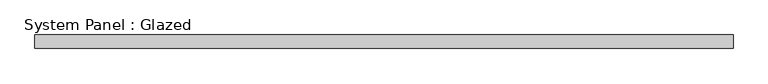
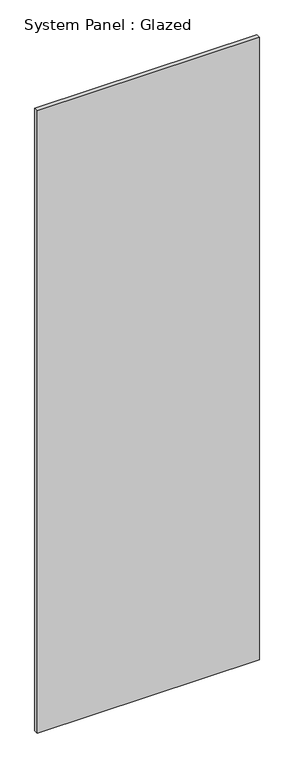
"""IFC4 building model written with IfcOpenShell, lengths in millimetres: plate geometry, System Panel : Glazed."""

import ifcopenshell
import ifcopenshell.guid

model = None  # the IFC model being written
_history = None  # IfcOwnerHistory: only IFC2X3 demands one
_inside = {}  # id of a spatial element -> (the spatial element, [elements in it])
_under = {}  # id of a project, library or spatial element -> (it, [spatial elements below it])
_declared = {}  # id of a project -> (the project, [libraries it declares])
_typed = {}  # id of a type object -> (the type object, [elements of that type])
_made_of = {}  # id of a material, layer set ... -> (it, [elements and type objects made of it])


def new_model(schema):
    """Start an empty IFC model of exactly this schema.

    Asked for "IFC4X3", IfcOpenShell would pick the latest addendum, in which some entities
    have other attributes; the version numbers below select the first issue.
    IFC2X3 requires an IfcOwnerHistory on every rooted entity: one is made here for all.
    """
    global model, _history
    if schema == "IFC4X3":
        model = ifcopenshell.file(schema_version=(4, 3, 0, 0))
    else:
        model = ifcopenshell.file(schema=schema)
    _inside.clear()
    _under.clear()
    _declared.clear()
    _typed.clear()
    _made_of.clear()
    _history = None
    if model.schema == "IFC2X3":
        org = make("IfcOrganization", Name="unknown")
        user = make(
            "IfcPersonAndOrganization",
            ThePerson=make("IfcPerson", FamilyName="unknown"),
            TheOrganization=org,
        )
        app = make(
            "IfcApplication",
            ApplicationDeveloper=org,
            Version="unknown",
            ApplicationFullName="unknown",
            ApplicationIdentifier="unknown",
        )
        _history = make(
            "IfcOwnerHistory",
            OwningUser=user,
            OwningApplication=app,
            ChangeAction="ADDED",
            CreationDate=0,
        )
    return model


def make(cls, **values):
    """One entity of the class cls with the attributes given. An attribute that is None is left unset."""
    return model.create_entity(
        cls, **{name: value for name, value in values.items() if value is not None}
    )


def rooted(cls, **values):
    """An entity with a GlobalId (a new one), such as an element, a storey or a relation."""
    return make(cls, GlobalId=ifcopenshell.guid.new(), OwnerHistory=_history, **values)


def si_unit(unit_type, name, prefix=None):
    """IfcSIUnit, for example si_unit("LENGTHUNIT", "METRE", prefix="MILLI")."""
    return make("IfcSIUnit", UnitType=unit_type, Prefix=prefix, Name=name)


def assignment(units):
    """IfcUnitAssignment: the units of a project."""
    return None if units is None else make("IfcUnitAssignment", Units=units)


def point(xyz):
    """IfcCartesianPoint."""
    return None if xyz is None else make("IfcCartesianPoint", Coordinates=xyz)


def direction(xyz):
    """IfcDirection."""
    return None if xyz is None else make("IfcDirection", DirectionRatios=xyz)


def frame(location, z_axis=None, x_axis=None):
    """IfcAxis2Placement3D, a coordinate frame: its origin and axes. An axis left out is left unset."""
    return make(
        "IfcAxis2Placement3D",
        Location=point(location),
        Axis=direction(z_axis),
        RefDirection=direction(x_axis),
    )


def origin():
    """The frame at (0, 0, 0) with its axes left unset."""
    return frame((0.0, 0.0, 0.0))


def origin_with_axes():
    """The frame at (0, 0, 0) with the z axis (0, 0, 1) and the x axis (1, 0, 0) written out."""
    return frame((0.0, 0.0, 0.0), z_axis=(0.0, 0.0, 1.0), x_axis=(1.0, 0.0, 0.0))


def place(relative_to, where):
    """IfcLocalPlacement: puts the frame where relative to a parent placement (None: the world)."""
    return make(
        "IfcLocalPlacement", PlacementRelTo=relative_to, RelativePlacement=where
    )


def context(
    kind, dimensions, precision=None, world=None, true_north=None, identifier=None
):
    """IfcGeometricRepresentationContext, for example the 3D "Model" context."""
    return make(
        "IfcGeometricRepresentationContext",
        ContextIdentifier=identifier,
        ContextType=kind,
        CoordinateSpaceDimension=dimensions,
        Precision=precision,
        WorldCoordinateSystem=world,
        TrueNorth=true_north,
    )


def project(units=None, contexts=None):
    """IfcProject with its units and contexts."""
    return rooted(
        "IfcProject",
        Name="project",
        RepresentationContexts=contexts,
        UnitsInContext=assignment(units),
    )


def spatial(cls, under=None, at=None, **own):
    """A site, building, storey or space (cls), placed at a placement, below another one or the project."""
    s = rooted(cls, ObjectPlacement=at, **own)
    if under is not None:
        _under.setdefault(under.id(), (under, []))[1].append(s)
    return s


def polyline(points):
    """IfcPolyline through the points."""
    return make("IfcPolyline", Points=[point(p) for p in points])


def outline(outer, holes=None, kind="AREA"):
    """IfcArbitraryClosedProfileDef: a profile drawn as a closed curve; with holes, ...WithVoids."""
    if holes is None:
        return make("IfcArbitraryClosedProfileDef", ProfileType=kind, OuterCurve=outer)
    return make(
        "IfcArbitraryProfileDefWithVoids",
        ProfileType=kind,
        OuterCurve=outer,
        InnerCurves=holes,
    )


def extrude(swept, where, along, depth):
    """IfcExtrudedAreaSolid: the profile swept, set in the frame where, extruded along a direction by depth."""
    return make(
        "IfcExtrudedAreaSolid",
        SweptArea=swept,
        Position=where,
        ExtrudedDirection=direction(along),
        Depth=depth,
    )


def shape(context_of_items, identifier, shape_type, items):
    """IfcShapeRepresentation: the items that make up one representation, for example the "Body"."""
    return make(
        "IfcShapeRepresentation",
        ContextOfItems=context_of_items,
        RepresentationIdentifier=identifier,
        RepresentationType=shape_type,
        Items=items,
    )


def source(mapping_origin, context_of_items, identifier, shape_type, items):
    """IfcRepresentationMap: a shape defined once, which mapped items show again and again."""
    return make(
        "IfcRepresentationMap",
        MappingOrigin=mapping_origin,
        MappedRepresentation=shape(context_of_items, identifier, shape_type, items),
    )


def transform(
    local_origin,
    x_axis=None,
    y_axis=None,
    z_axis=None,
    scale=None,
    scale2=None,
    scale3=None,
    uniform=True,
):
    """IfcCartesianTransformationOperator3D, or its non-uniform kind. x_axis, y_axis, z_axis: its Axis1, 2, 3."""
    if uniform:
        return make(
            "IfcCartesianTransformationOperator3D",
            Axis1=direction(x_axis),
            Axis2=direction(y_axis),
            LocalOrigin=point(local_origin),
            Scale=scale,
            Axis3=direction(z_axis),
        )
    return make(
        "IfcCartesianTransformationOperator3DnonUniform",
        Axis1=direction(x_axis),
        Axis2=direction(y_axis),
        LocalOrigin=point(local_origin),
        Scale=scale,
        Axis3=direction(z_axis),
        Scale2=scale2,
        Scale3=scale3,
    )


def mapped(mapping_source, mapping_target):
    """IfcMappedItem: shows the shape of a source again, moved by a transform."""
    return make(
        "IfcMappedItem", MappingSource=mapping_source, MappingTarget=mapping_target
    )


def made_of(thing, what):
    """Note that an element or type object is made of a material, layer set ...; save() writes the relation."""
    if what is not None:
        _made_of.setdefault(what.id(), (what, []))[1].append(thing)
    return thing


def element(
    cls,
    number,
    at=None,
    inside=None,
    cuts=None,
    type_object=None,
    material=None,
    context=None,
    identifier="Body",
    shape_type=None,
    held_by="IfcProductDefinitionShape",
    body=None,
    shapes=None,
    **own,
):
    """One element of the class cls, such as IfcWall. Its Tag is "e" and its number.

    at: its placement. inside: the storey or other place that contains it. cuts: it is an
    opening in that element (IfcRelVoidsElement). A single representation is given by context,
    identifier, shape_type and body (its items); several are given by shapes. held_by: the class
    of the entity that holds the representations. save() writes the other relations.
    """
    e = rooted(cls, Tag="e%d" % number, ObjectPlacement=at, **own)
    if body is not None:
        shapes = [shape(context, identifier, shape_type, body)]
    if shapes is not None:
        e.Representation = make(held_by, Representations=shapes)
    if inside is not None:
        _inside.setdefault(inside.id(), (inside, []))[1].append(e)
    if cuts is not None:
        rooted(
            "IfcRelVoidsElement", RelatingBuildingElement=cuts, RelatedOpeningElement=e
        )
    if type_object is not None:
        _typed.setdefault(type_object.id(), (type_object, []))[1].append(e)
    return made_of(e, material)


def aggregate(whole, parts):
    """IfcRelAggregates: a whole, such as a stair, and the parts it consists of."""
    return rooted("IfcRelAggregates", RelatingObject=whole, RelatedObjects=parts)


def save(model, path):
    """Write the relations noted so far, then the file.

    IfcRelAggregates (storeys below a building ...), IfcRelContainedInSpatialStructure (elements
    in a storey), IfcRelDefinesByType, IfcRelAssociatesMaterial and IfcRelDeclares: one each for
    every whole, place, type object, material and project.
    """
    for whole, parts in _under.values():
        aggregate(whole, parts)
    for where, things in _inside.values():
        rooted(
            "IfcRelContainedInSpatialStructure",
            RelatedElements=things,
            RelatingStructure=where,
        )
    for kind, things in _typed.values():
        rooted("IfcRelDefinesByType", RelatedObjects=things, RelatingType=kind)
    for what, things in _made_of.values():
        rooted("IfcRelAssociatesMaterial", RelatedObjects=things, RelatingMaterial=what)
    for by, libraries in _declared.values():
        rooted("IfcRelDeclares", RelatingContext=by, RelatedDefinitions=libraries)
    model.write(path)


def system_panel_glazed_f91df05e(model_context):
    return source(origin(), model_context, "Body", "SweptSolid", [
        extrude(outline(polyline([(660.033654, 19.05), (-660.033654, 19.05), (-660.033654, 44.45), (660.033654, 44.45), (660.033654, 19.05)])), origin_with_axes(), (0.0, 0.0, 1.0), 3908.2835741),
    ])


if __name__ == "__main__":
    model = new_model("IFC4")
    model_context = context("Model", 3, world=origin())
    ifc_project = project(units=[si_unit("LENGTHUNIT", "METRE", prefix="MILLI")], contexts=[model_context])
    site = spatial("IfcSite", under=ifc_project)
    building = spatial("IfcBuilding", under=site)
    placement = place(None, origin())
    system_panel_glazed_shape = system_panel_glazed_f91df05e(model_context)
    element("IfcPlate", 1, ObjectType="System Panel : Glazed", at=placement, inside=building, context=model_context, shape_type="MappedRepresentation", body=[
        mapped(system_panel_glazed_shape, transform((0.0, 0.0, 0.0), x_axis=(1.0, 0.0, 0.0), y_axis=(0.0, 1.0, 0.0), z_axis=(0.0, 0.0, 1.0))),
    ])
    save(model, "model.ifc")

# Revit data of these elements
# Type "System Panel : Glazed"
#   Construction Type Id = "GSP4R"
#   Analytic Construction = "1/8 in Pilkington single glazing"
#   Visual Light Transmittance = 0.9
#   Solar Heat Gain Coefficient = 0.86
#   Heat Transfer Coefficient (U) = 1.18115 BTU/(h·ft²·°F)
#   Define Thermal Properties by = 1
# Element 1 (IfcPlate, "System Panel : Glazed")
#   Materials on its faces: "Glass"
# Materials
#   "Glass": class "Glass", colour RGB 0 128 192, transparency 0.75, Description = "Soda Lime Glass", Cost = 0
